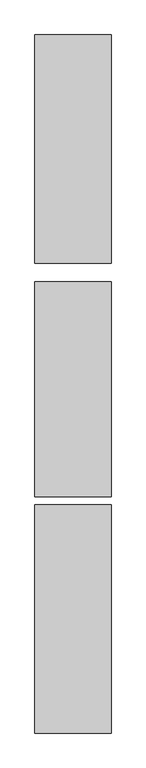
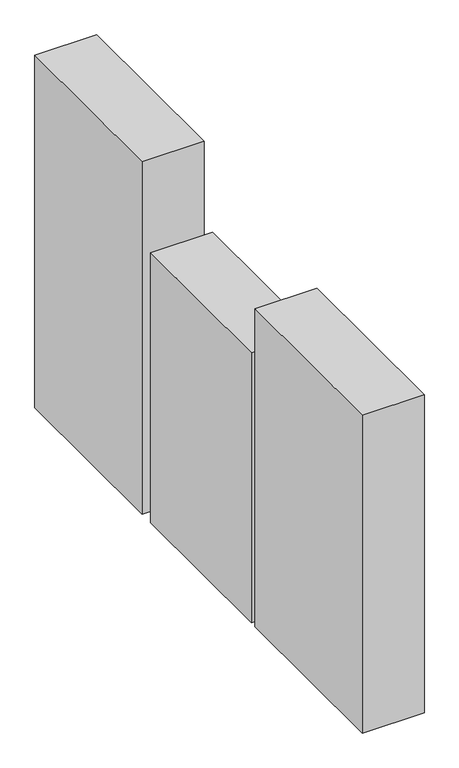
"""IFC4 building model written with IfcOpenShell, lengths in millimetres: furniture geometry, Metalic shelf : Metalic shelf."""

from ifc_helpers import new_model, si_unit, origin, origin_with_axes, place, context, project, spatial, polyline, outline, extrude, source, transform, mapped, element, save


def furniture_03baebca(model_context):
    return source(origin(), model_context, "Body", "SweptSolid", [
        extrude(outline(polyline([(23330.6870052, 5077.1180714), (23635.4870052, 5077.1180714), (23635.4870052, 4217.6615366), (23330.6870052, 4217.6615366), (23330.6870052, 5077.1180714)])), origin_with_axes(), (0.0, 0.0, 1.0), 1406.0770761),
        extrude(outline(polyline([(23635.4870052, 3271.5115366), (23330.6870052, 3271.5115366), (23330.6870052, 4185.9115366), (23635.4870052, 4185.9115366), (23635.4870052, 3271.5115366)])), origin_with_axes(), (0.0, 0.0, 1.0), 1653.2066023),
        extrude(outline(polyline([(23635.4870052, 5151.1115366), (23330.6870052, 5151.1115366), (23330.6870052, 6065.5115366), (23635.4870052, 6065.5115366), (23635.4870052, 5151.1115366)])), origin_with_axes(), (0.0, 0.0, 1.0), 1832.7434172),
    ])


if __name__ == "__main__":
    model = new_model("IFC4")
    model_context = context("Model", 3, world=origin())
    ifc_project = project(units=[si_unit("LENGTHUNIT", "METRE", prefix="MILLI")], contexts=[model_context])
    site = spatial("IfcSite", under=ifc_project)
    building = spatial("IfcBuilding", under=site)
    placement = place(None, origin())
    furniture_shape = furniture_03baebca(model_context)
    element("IfcFurniture", 1, ObjectType="Metalic shelf : Metalic shelf", at=placement, inside=building, context=model_context, shape_type="MappedRepresentation", body=[
        mapped(furniture_shape, transform((0.0, 0.0, 0.0), x_axis=(1.0, 0.0, 0.0), y_axis=(0.0, 1.0, 0.0), z_axis=(0.0, 0.0, 1.0))),
    ])
    save(model, "model.ifc")

# Revit data of these elements
# Element 1 (IfcFurniture, "Metalic shelf : Metalic shelf")
#   Materials on its faces: "food"
# Materials
#   "food": class "Glass", colour RGB 233 233 233, transparency 0, Description = "Soda Lime Glass", Cost = 0
